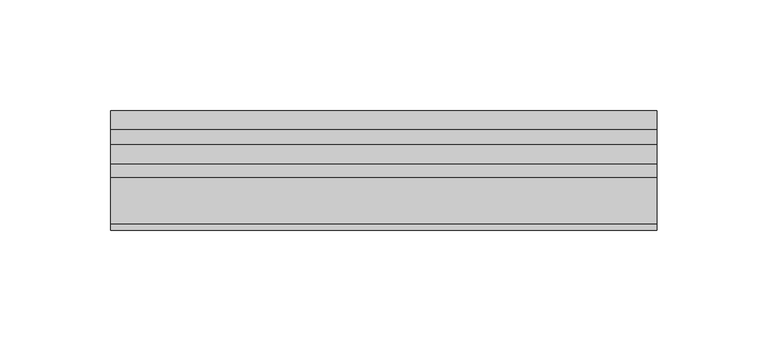
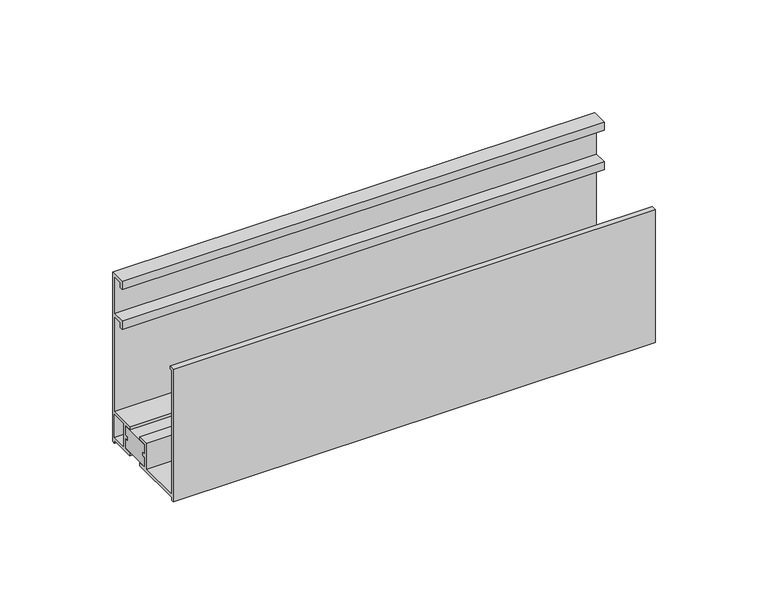
"""IFC4 building model written with IfcOpenShell, lengths in millimetres: proxy geometry, Generic Models 2:Generic Models 2:310765:Generic Models 2:310765 : Generic Models 2:Generic Models 2:310765:68 : Generic Models 2:Generic Models 2:310765:Generic Models 2:310765 : Generic Models 2:Generic Models 2:310765:300385."""

from ifc_helpers import new_model, si_unit, frame, origin, place, context, project, spatial, polyline, outline, extrude, source, transform, mapped, element, save


def generic_models_dad187ab(model_context):
    return source(origin(), model_context, "Body", "SweptSolid", [
        extrude(outline(polyline([(-16.5522562, 0.0), (0.0, 0.0), (0.0, -4.6974986), (-1.9254154, -4.6974986), (-1.9254154, -7.0787486), (0.0, -7.0787486), (0.0, -11.7762472), (-16.5522562, -11.7762472), (-16.5522562, -7.0787486), (-14.6268407, -7.0787486), (-14.6268407, -4.6974986), (-16.5522562, -4.6974986), (-16.5522562, 0.0)])), frame((667295.8649872, -568229.8645058, 6212.1988969), z_axis=(1.0, 0.0, 4.195754854663392e-12), x_axis=(0.0, 1.0, 0.0)), (0.0, 0.0, 1.0), 247.0688117),
        extrude(outline(polyline([(-8.4463715, 0.0), (0.0, 0.0), (0.0, -92.0), (-1.5875, -92.0), (-1.5875, -90.4125), (-15.2853225, -90.4125), (-15.2853225, -88.825), (-11.118135, -88.825), (-11.118135, -83.3337514), (-13.0435504, -83.3337514), (-13.0435504, -81.7462514), (-11.118135, -81.7462514), (-11.118135, -76.2550028), (-15.2853225, -76.2550028), (-15.2853225, -74.6675028), (-1.5875, -74.6675028), (-1.5875, -23.175), (-6.8588715, -23.175), (-6.8588715, -25.9748266), (-8.4463715, -25.9748266), (-8.4463715, -21.5875), (-1.5875, -21.5875), (-1.5875, -1.5875), (-6.8588715, -1.5875), (-6.8588715, -4.3873266), (-8.4463715, -4.3873266), (-8.4463715, 0.0)]), holes=[polyline([(-1.5875, -76.2550028), (-9.530635, -76.2550028), (-9.530635, -88.825), (-1.5875, -88.825), (-1.5875, -76.2550028)])]), frame((667295.8649872, -568218.3494958, 6288.8507747), z_axis=(1.0, 0.0, 4.195754854663392e-12), x_axis=(0.0, 1.0, 0.0)), (0.0, 0.0, 1.0), 247.0688117),
        extrude(outline(polyline([(-1.5875, 0.0), (0.0, 0.0), (0.0, -72.0), (-2.7150899, -72.0), (-2.7150899, -70.4125), (-1.5875, -70.4125), (-1.5875, -3.175), (-23.9483588, -3.175), (-23.9483588, -17.3324972), (-29.7030463, -17.3324972), (-29.7030463, -15.7449972), (-25.5358588, -15.7449972), (-25.5358588, -10.2537486), (-27.4612743, -10.2537486), (-27.4612743, -8.6662486), (-25.5358588, -8.6662486), (-25.5358588, -3.175), (-29.7030463, -3.175), (-29.7030463, -1.5875), (-1.5875, -1.5875), (-1.5875, 0.0)])), frame((667295.8649872, -568272.3494958, 6196.8507747), z_axis=(1.0, 0.0, 4.195754854663392e-12), x_axis=(0.0, -1.0, 0.0)), (0.0, 0.0, 1.0), 247.0688117),
    ])


if __name__ == "__main__":
    model = new_model("IFC4")
    model_context = context("Model", 3, world=origin())
    ifc_project = project(units=[si_unit("LENGTHUNIT", "METRE", prefix="MILLI")], contexts=[model_context])
    site = spatial("IfcSite", under=ifc_project)
    building = spatial("IfcBuilding", under=site)
    placement = place(None, origin())
    generic_models_shape = generic_models_dad187ab(model_context)
    element("IfcBuildingElementProxy", 1, Name="Generic Models 2:Generic Models 2:310765:Generic Models 2:310765 : Generic Models 2:Generic Models 2:310765:68 : Generic Models 2:Generic Models 2:310765:Generic Models 2:310765 : Generic Models 2:Generic Models 2:310765:300385", ObjectType="Generic Models 2:Generic Models 2:310765:Generic Models 2:310765 : Generic Models 2:Generic Models 2:310765:68 : Generic Models 2:Generic Models 2:310765:Generic Models 2:310765 : Generic Models 2:Generic Models 2:310765:300385", at=placement, inside=building, context=model_context, shape_type="MappedRepresentation", body=[
        mapped(generic_models_shape, transform((0.0, 0.0, 0.0), x_axis=(1.0, 0.0, 0.0), y_axis=(0.0, 1.0, 0.0), z_axis=(0.0, 0.0, 1.0))),
    ])
    save(model, "model.ifc")

# Revit data of these elements
# Type "Generic Models 2:Generic Models 2:310765:Generic Models 2:310765 : Generic Models 2:Generic Models 2:310765:68 : Generic Models 2:Generic Models 2:310765:Generic Models 2:310765 : Generic Models 2:Generic Models 2:310765:300385"
#   NameOverride = "Generic Models 2:Generic Models 2:310765:Generic Models 2:310765 : Generic Models 2:Generic Models 2:310765:300385"
#   ObjectTypeOverride = "Generic Models 2:310765 : Generic Models 2:Generic Models 2:310765"
#   Reference = "Generic Models 2"
#   Tag = "300385"
# Element 1 (IfcBuildingElementProxy, "Generic Models 2:Generic Models 2:310765:Generic Models 2:310765 : Generic Models 2:Generic Models 2:310765:68 : Generic Models 2:Generic Models 2:310765:Generic Models 2:310765 : Generic Models 2:Generic Models 2:310765:300385")
#   Materials on its faces: "THERMAL BROKEN ALUMINUM STOREFRONT FOR POLYCARBONATE"
# Materials
#   "THERMAL BROKEN ALUMINUM STOREFRONT FOR POLYCARBONATE": class "Unassigned", colour RGB 244 244 244, transparency 0, Keynote = "M07611300.01", Cost = 0
